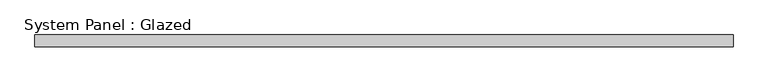
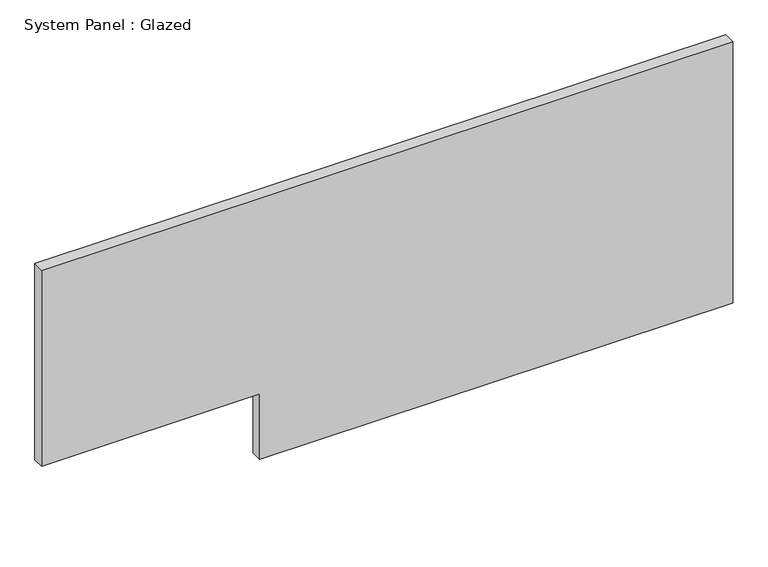
"""IFC4 building model written with IfcOpenShell, lengths in millimetres: plate geometry, System Panel : Glazed."""

from ifc_helpers import new_model, si_unit, frame, origin, place, context, project, spatial, polyline, outline, extrude, source, transform, mapped, element, save


def system_panel_glazed_4337754e(model_context):
    return source(origin(), model_context, "Body", "SweptSolid", [
        extrude(outline(polyline([(0.0, -281.0287927), (0.0, 762.0), (609.6, 762.0), (609.6, -762.0), (152.4, -762.0), (152.4, -281.0287927), (0.0, -281.0287927)])), frame((0.0, 19.05, 0.0), z_axis=(0.0, 1.0, 0.0), x_axis=(0.0, 0.0, 1.0)), (0.0, 0.0, 1.0), 25.4),
    ])


if __name__ == "__main__":
    model = new_model("IFC4")
    model_context = context("Model", 3, world=origin())
    ifc_project = project(units=[si_unit("LENGTHUNIT", "METRE", prefix="MILLI")], contexts=[model_context])
    site = spatial("IfcSite", under=ifc_project)
    building = spatial("IfcBuilding", under=site)
    placement = place(None, origin())
    system_panel_glazed_shape = system_panel_glazed_4337754e(model_context)
    element("IfcPlate", 1, ObjectType="System Panel : Glazed", at=placement, inside=building, context=model_context, shape_type="MappedRepresentation", body=[
        mapped(system_panel_glazed_shape, transform((0.0, 0.0, 0.0), x_axis=(1.0, 0.0, 0.0), y_axis=(0.0, 1.0, 0.0), z_axis=(0.0, 0.0, 1.0))),
    ])
    save(model, "model.ifc")

# Revit data of these elements
# Element 1 (IfcPlate, "System Panel : Glazed")
#   Materials on its faces: "Glass"
# Materials
#   "Glass": class "Glass", colour RGB 0 128 192, transparency 0.75
